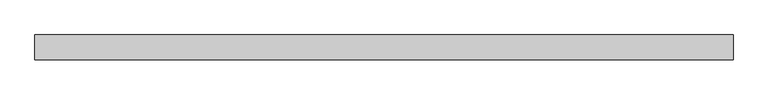
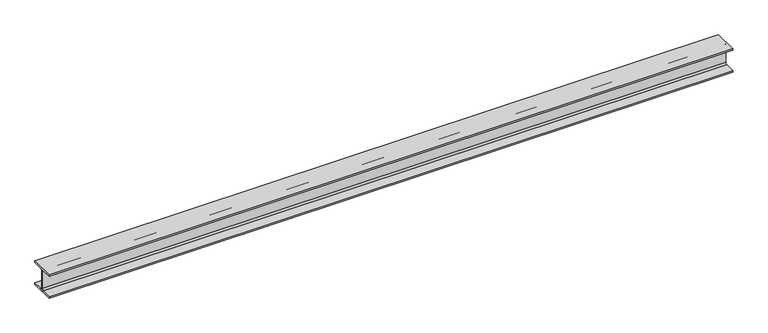
"""IFC4 building model written with IfcOpenShell, lengths in millimetres: beam geometry, 0912_Steel Framing_H-KSD3502 : H_SB_ASB_H-200x200x8x12."""

from ifc_helpers import new_model, si_unit, point, frame, frame_2d, origin, place, context, project, spatial, polyline, circle_curve, trimmed, segment, composite_curve, outline, extrude, source, transform, mapped, element, save


def beam_6e275dda(model_context):
    return source(origin(), model_context, "Body", "SweptSolid", [
        extrude(outline(composite_curve([segment(polyline([(100.0, -88.0), (100.0, -100.0), (-100.0, -100.0), (-100.0, -88.0), (-17.0, -88.0)]), True, "CONTINUOUS"), segment(trimmed(circle_curve(frame_2d((-17.0, -75.0)), 13.0), [point((-17.0, -88.0))], [point((-4.0, -75.0))], True, "CARTESIAN"), True, "CONTINUOUS"), segment(polyline([(-4.0, -75.0), (-4.0, 75.0)]), True, "CONTINUOUS"), segment(trimmed(circle_curve(frame_2d((-17.0, 75.0)), 13.0), [point((-4.0, 75.0))], [point((-17.0, 88.0))], True, "CARTESIAN"), True, "CONTINUOUS"), segment(polyline([(-17.0, 88.0), (-100.0, 88.0), (-100.0, 100.0), (100.0, 100.0), (100.0, 88.0), (17.0, 88.0)]), True, "CONTINUOUS"), segment(trimmed(circle_curve(frame_2d((17.0, 75.0)), 13.0), [point((17.0, 88.0))], [point((4.0, 75.0))], True, "CARTESIAN"), True, "CONTINUOUS"), segment(polyline([(4.0, 75.0), (4.0, -75.0)]), True, "CONTINUOUS"), segment(trimmed(circle_curve(frame_2d((17.0, -75.0)), 13.0), [point((4.0, -75.0))], [point((17.0, -88.0))], True, "CARTESIAN"), True, "CONTINUOUS"), segment(polyline([(17.0, -88.0), (100.0, -88.0)]), True, "CONTINUOUS")], self_intersect=False)), frame((-2922.8724307, 0.0, 0.0), z_axis=(1.0, 0.0, 0.0), x_axis=(0.0, 1.0, 0.0)), (0.0, 0.0, 1.0), 5598.8679606),
    ])


if __name__ == "__main__":
    model = new_model("IFC4")
    model_context = context("Model", 3, world=origin())
    ifc_project = project(units=[si_unit("LENGTHUNIT", "METRE", prefix="MILLI")], contexts=[model_context])
    site = spatial("IfcSite", under=ifc_project)
    building = spatial("IfcBuilding", under=site)
    placement = place(None, origin())
    beam_shape = beam_6e275dda(model_context)
    element("IfcBeam", 1, ObjectType="0912_Steel Framing_H-KSD3502 : H_SB_ASB_H-200x200x8x12", at=placement, inside=building, context=model_context, shape_type="MappedRepresentation", body=[
        mapped(beam_shape, transform((0.0, 0.0, 0.0), x_axis=(1.0, 0.0, 0.0), y_axis=(0.0, 1.0, 0.0), z_axis=(0.0, 0.0, 1.0))),
    ])
    save(model, "model.ifc")

# Revit data of these elements
# Type "0912_Steel Framing_H-KSD3502 : H_SB_ASB_H-200x200x8x12"
#   H_WM Code_1 = "S01AA002-00001 | Main Steel Structure Fabrication Work | Shelter/Building | Medium Steel - Standard (90KG/M>Weight≥30KG/M) | Material: (   )"
#   H_WM Code_2 = "S03AA028-00001 | Main Steel Structure Erection Work | Shelter/Building | Medium Steel (90KG/M>Weight≥30KG/M) | Material: (   )"
#   H_WM Code_3 = "S01AA010-00001 | Main Steel Structure Fabrication Work | Shelter/Building | Steel Painting/Coating | for Non-Fireproofed Steel Surface, Surface Preparation, Primer, Second & Final Coat | Material: (   )"
#   H_Q'ty Cal Type Tag = "SB-Q2"
#   Width = 20.0 cm
#   Web Thickness = 0.8 cm
#   Web Fillet = 1.3 cm
#   Warping Constant = 141000.0 cm⁶
#   W = 0
#   Torsional Moment of Inertia = 26.2485 cm⁴
#   Section Area = 63.53 cm²
#   Plastic Modulus weak axis = 244.0 cm³
#   Plastic Modulus strong axis = 525.0 cm³
#   Perimeter = 1.16 m²/m
#   Nominal Weight = 49.90 kgf/m
#   Moment of Inertia weak axis = 1600.00 cm⁴
#   Moment of Inertia strong axis = 4720.00 cm⁴
#   Height = 20.0 cm
#   Flange Thickness = 1.2 cm
#   Elastic Modulus weak axis = 160.0 cm³
#   Elastic Modulus strong axis = 472.0 cm³
#   Centroid Vertical = 10.0 cm
#   Centroid Horizontal = 10.0 cm
#   Ix = 47200000
#   Length [instance default] = 1.5240 m
#   Zx = 525000
#   b = 0.2000 m
#   h = 0.2000 m
#   r = 0.0130 m
#   s = 0.0080 m
#   t = 0.0120 m
#   A = 0.006353 m²
#   Structural Material [instance default] = Steel, 45-345
#   Assembly Code = ""
# Element 1 (IfcBeam, "0912_Steel Framing_H-KSD3502 : H_SB_ASB_H-200x200x8x12")
#   Structural Material = none
# Materials
#   "Steel, 45-345": class "Metal", colour RGB 189 187 185, transparency 0, Description = "Steel 345 MPa", Cost = 0
